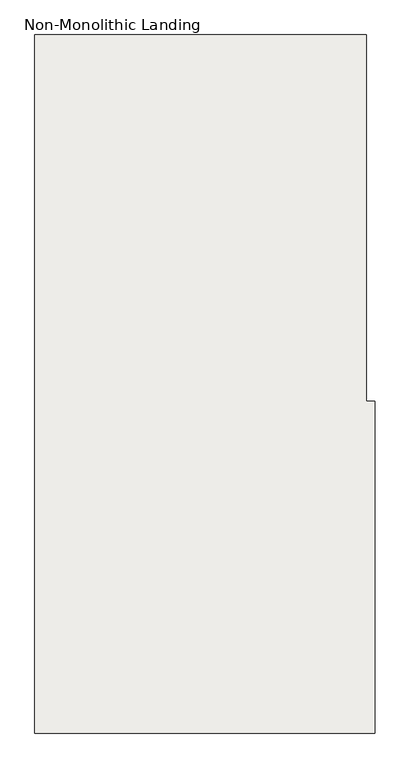
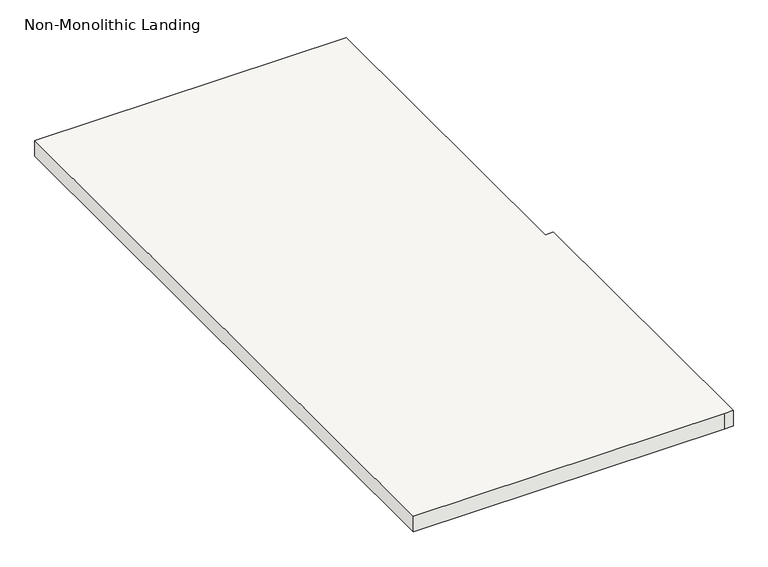
"""IFC4 building model written with IfcOpenShell, lengths in millimetres: slab geometry, Non-Monolithic Landing."""

from ifc_helpers import new_model, si_unit, origin, place, context, project, spatial, faceted_brep, source, transform, mapped, element, save


def non_monolithic_landing_f03c976a(model_context):
    return source(origin(), model_context, "Body", "Brep", [
        faceted_brep([(24782.4590778, 27767.6156612, 267754.1), (24807.8590778, 27767.6156612, 267779.5), (24807.8590778, 26802.4156612, 267779.5), (24782.4590778, 26802.4156612, 267754.1), (23842.6590778, 27767.6156612, 267798.55), (23842.6590778, 25735.6156612, 267798.55), (24807.8590778, 25735.6156612, 267798.55), (24833.2590778, 25735.6156612, 267798.55), (24833.2590778, 26700.8156612, 267798.55), (24807.8590778, 26700.8156612, 267798.55), (24807.8590778, 27767.6156612, 267798.55), (24782.4590778, 26802.4156612, 267747.75), (24807.8590778, 26802.4156612, 267747.75), (24807.8590778, 26700.8156612, 267747.75), (24833.2590778, 26700.8156612, 267747.75), (24833.2590778, 25735.6156612, 267747.75), (24807.8590778, 25735.6156612, 267747.75), (23842.6590778, 25735.6156612, 267747.75), (23842.6590778, 27767.6156612, 267747.75), (24782.4590778, 27767.6156612, 267747.75)], [[[0, 1, 2, 3]], [[4, 5, 6, 7, 8, 9, 10]], [[11, 12, 13, 14, 15, 16, 17, 18, 19]], [[11, 19, 0, 3]], [[10, 9, 13, 12, 2, 1]], [[8, 7, 15, 14]], [[7, 6, 16, 15]], [[6, 5, 17, 16]], [[5, 4, 18, 17]], [[4, 10, 1, 0, 19, 18]], [[12, 11, 3, 2]], [[9, 8, 14, 13]]]),
    ])


if __name__ == "__main__":
    model = new_model("IFC4")
    model_context = context("Model", 3, world=origin())
    ifc_project = project(units=[si_unit("LENGTHUNIT", "METRE", prefix="MILLI")], contexts=[model_context])
    site = spatial("IfcSite", under=ifc_project)
    building = spatial("IfcBuilding", under=site)
    placement = place(None, origin())
    non_monolithic_landing_shape = non_monolithic_landing_f03c976a(model_context)
    element("IfcSlab", 1, ObjectType="Non-Monolithic Landing", at=placement, inside=building, context=model_context, shape_type="MappedRepresentation", body=[
        mapped(non_monolithic_landing_shape, transform((0.0, 0.0, 0.0), x_axis=(1.0, 0.0, 0.0), y_axis=(0.0, 1.0, 0.0), z_axis=(0.0, 0.0, 1.0))),
    ])
    save(model, "model.ifc")

# Revit data of these elements
# Element 1 (IfcSlab, "Non-Monolithic Landing")
#   Materials on its faces: "SLOTTED WOOD FENCE (THERMALLY MODIFIED WOOD: ARBOR WOOD)\n(EXTERIOR STAIN : PENOFIN VERDE EXT. STAIN - COLOR: CEDAR)"
# Materials
#   "SLOTTED WOOD FENCE (THERMALLY MODIFIED WOOD: ARBOR WOOD)\n(EXTERIOR STAIN : PENOFIN VERDE EXT. STAIN - COLOR: CEDAR)": class "Wood", colour RGB 164 134 123, transparency 0, Description = "Pinus Echinata", Cost = 0
